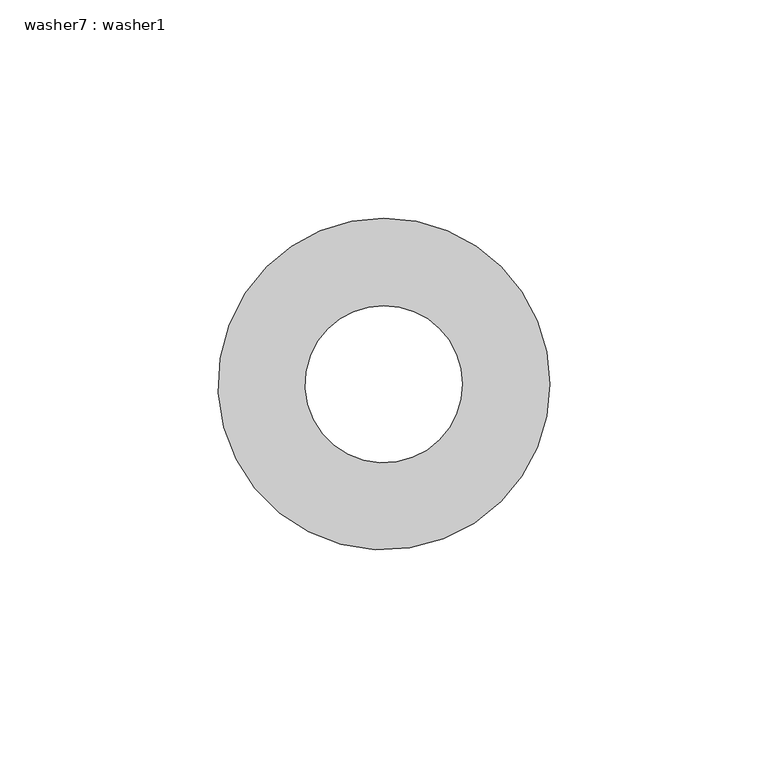
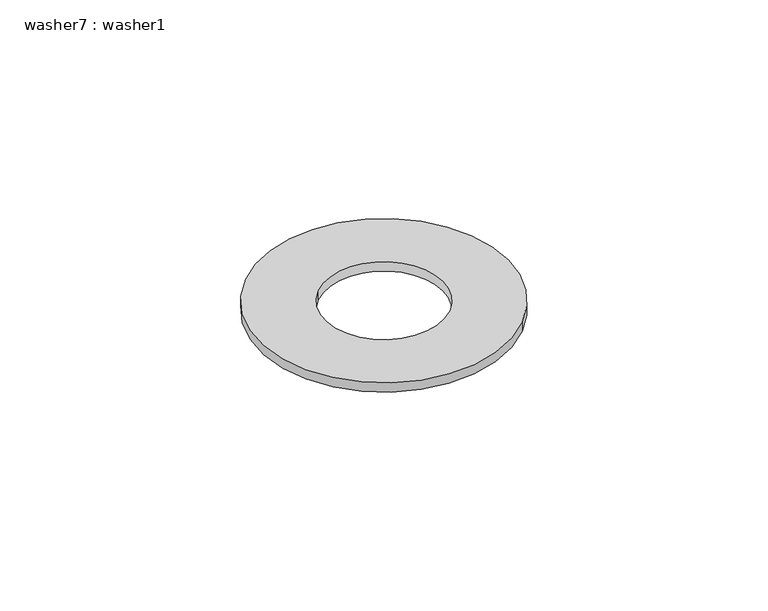
"""IFC4 building model written with IfcOpenShell, lengths in millimetres: fastener geometry, washer7 : washer1."""

import ifcopenshell
import ifcopenshell.guid

model = None  # the IFC model being written
_history = None  # IfcOwnerHistory: only IFC2X3 demands one
_inside = {}  # id of a spatial element -> (the spatial element, [elements in it])
_under = {}  # id of a project, library or spatial element -> (it, [spatial elements below it])
_declared = {}  # id of a project -> (the project, [libraries it declares])
_typed = {}  # id of a type object -> (the type object, [elements of that type])
_made_of = {}  # id of a material, layer set ... -> (it, [elements and type objects made of it])


def new_model(schema):
    """Start an empty IFC model of exactly this schema.

    Asked for "IFC4X3", IfcOpenShell would pick the latest addendum, in which some entities
    have other attributes; the version numbers below select the first issue.
    IFC2X3 requires an IfcOwnerHistory on every rooted entity: one is made here for all.
    """
    global model, _history
    if schema == "IFC4X3":
        model = ifcopenshell.file(schema_version=(4, 3, 0, 0))
    else:
        model = ifcopenshell.file(schema=schema)
    _inside.clear()
    _under.clear()
    _declared.clear()
    _typed.clear()
    _made_of.clear()
    _history = None
    if model.schema == "IFC2X3":
        org = make("IfcOrganization", Name="unknown")
        user = make(
            "IfcPersonAndOrganization",
            ThePerson=make("IfcPerson", FamilyName="unknown"),
            TheOrganization=org,
        )
        app = make(
            "IfcApplication",
            ApplicationDeveloper=org,
            Version="unknown",
            ApplicationFullName="unknown",
            ApplicationIdentifier="unknown",
        )
        _history = make(
            "IfcOwnerHistory",
            OwningUser=user,
            OwningApplication=app,
            ChangeAction="ADDED",
            CreationDate=0,
        )
    return model


def make(cls, **values):
    """One entity of the class cls with the attributes given. An attribute that is None is left unset."""
    return model.create_entity(
        cls, **{name: value for name, value in values.items() if value is not None}
    )


def rooted(cls, **values):
    """An entity with a GlobalId (a new one), such as an element, a storey or a relation."""
    return make(cls, GlobalId=ifcopenshell.guid.new(), OwnerHistory=_history, **values)


def si_unit(unit_type, name, prefix=None):
    """IfcSIUnit, for example si_unit("LENGTHUNIT", "METRE", prefix="MILLI")."""
    return make("IfcSIUnit", UnitType=unit_type, Prefix=prefix, Name=name)


def assignment(units):
    """IfcUnitAssignment: the units of a project."""
    return None if units is None else make("IfcUnitAssignment", Units=units)


def point(xyz):
    """IfcCartesianPoint."""
    return None if xyz is None else make("IfcCartesianPoint", Coordinates=xyz)


def direction(xyz):
    """IfcDirection."""
    return None if xyz is None else make("IfcDirection", DirectionRatios=xyz)


def frame(location, z_axis=None, x_axis=None):
    """IfcAxis2Placement3D, a coordinate frame: its origin and axes. An axis left out is left unset."""
    return make(
        "IfcAxis2Placement3D",
        Location=point(location),
        Axis=direction(z_axis),
        RefDirection=direction(x_axis),
    )


def frame_2d(location, x_axis=None):
    """IfcAxis2Placement2D, a coordinate frame in the plane: its origin and x axis."""
    return make(
        "IfcAxis2Placement2D", Location=point(location), RefDirection=direction(x_axis)
    )


def origin():
    """The frame at (0, 0, 0) with its axes left unset."""
    return frame((0.0, 0.0, 0.0))


def place(relative_to, where):
    """IfcLocalPlacement: puts the frame where relative to a parent placement (None: the world)."""
    return make(
        "IfcLocalPlacement", PlacementRelTo=relative_to, RelativePlacement=where
    )


def context(
    kind, dimensions, precision=None, world=None, true_north=None, identifier=None
):
    """IfcGeometricRepresentationContext, for example the 3D "Model" context."""
    return make(
        "IfcGeometricRepresentationContext",
        ContextIdentifier=identifier,
        ContextType=kind,
        CoordinateSpaceDimension=dimensions,
        Precision=precision,
        WorldCoordinateSystem=world,
        TrueNorth=true_north,
    )


def project(units=None, contexts=None):
    """IfcProject with its units and contexts."""
    return rooted(
        "IfcProject",
        Name="project",
        RepresentationContexts=contexts,
        UnitsInContext=assignment(units),
    )


def spatial(cls, under=None, at=None, **own):
    """A site, building, storey or space (cls), placed at a placement, below another one or the project."""
    s = rooted(cls, ObjectPlacement=at, **own)
    if under is not None:
        _under.setdefault(under.id(), (under, []))[1].append(s)
    return s


def circle_curve(where, radius):
    """IfcCircle in the frame where."""
    return make("IfcCircle", Position=where, Radius=radius)


def trimmed(basis, trim1, trim2, sense, master):
    """IfcTrimmedCurve: the piece of a basis curve between two trims."""
    return make(
        "IfcTrimmedCurve",
        BasisCurve=basis,
        Trim1=trim1,
        Trim2=trim2,
        SenseAgreement=sense,
        MasterRepresentation=master,
    )


def segment(curve, same_sense, transition):
    """IfcCompositeCurveSegment."""
    return make(
        "IfcCompositeCurveSegment",
        Transition=transition,
        SameSense=same_sense,
        ParentCurve=curve,
    )


def composite_curve(segments, self_intersect=None):
    """IfcCompositeCurve: segments joined end to end."""
    return make("IfcCompositeCurve", Segments=segments, SelfIntersect=self_intersect)


def outline(outer, holes=None, kind="AREA"):
    """IfcArbitraryClosedProfileDef: a profile drawn as a closed curve; with holes, ...WithVoids."""
    if holes is None:
        return make("IfcArbitraryClosedProfileDef", ProfileType=kind, OuterCurve=outer)
    return make(
        "IfcArbitraryProfileDefWithVoids",
        ProfileType=kind,
        OuterCurve=outer,
        InnerCurves=holes,
    )


def extrude(swept, where, along, depth):
    """IfcExtrudedAreaSolid: the profile swept, set in the frame where, extruded along a direction by depth."""
    return make(
        "IfcExtrudedAreaSolid",
        SweptArea=swept,
        Position=where,
        ExtrudedDirection=direction(along),
        Depth=depth,
    )


def shape(context_of_items, identifier, shape_type, items):
    """IfcShapeRepresentation: the items that make up one representation, for example the "Body"."""
    return make(
        "IfcShapeRepresentation",
        ContextOfItems=context_of_items,
        RepresentationIdentifier=identifier,
        RepresentationType=shape_type,
        Items=items,
    )


def source(mapping_origin, context_of_items, identifier, shape_type, items):
    """IfcRepresentationMap: a shape defined once, which mapped items show again and again."""
    return make(
        "IfcRepresentationMap",
        MappingOrigin=mapping_origin,
        MappedRepresentation=shape(context_of_items, identifier, shape_type, items),
    )


def transform(
    local_origin,
    x_axis=None,
    y_axis=None,
    z_axis=None,
    scale=None,
    scale2=None,
    scale3=None,
    uniform=True,
):
    """IfcCartesianTransformationOperator3D, or its non-uniform kind. x_axis, y_axis, z_axis: its Axis1, 2, 3."""
    if uniform:
        return make(
            "IfcCartesianTransformationOperator3D",
            Axis1=direction(x_axis),
            Axis2=direction(y_axis),
            LocalOrigin=point(local_origin),
            Scale=scale,
            Axis3=direction(z_axis),
        )
    return make(
        "IfcCartesianTransformationOperator3DnonUniform",
        Axis1=direction(x_axis),
        Axis2=direction(y_axis),
        LocalOrigin=point(local_origin),
        Scale=scale,
        Axis3=direction(z_axis),
        Scale2=scale2,
        Scale3=scale3,
    )


def mapped(mapping_source, mapping_target):
    """IfcMappedItem: shows the shape of a source again, moved by a transform."""
    return make(
        "IfcMappedItem", MappingSource=mapping_source, MappingTarget=mapping_target
    )


def made_of(thing, what):
    """Note that an element or type object is made of a material, layer set ...; save() writes the relation."""
    if what is not None:
        _made_of.setdefault(what.id(), (what, []))[1].append(thing)
    return thing


def element(
    cls,
    number,
    at=None,
    inside=None,
    cuts=None,
    type_object=None,
    material=None,
    context=None,
    identifier="Body",
    shape_type=None,
    held_by="IfcProductDefinitionShape",
    body=None,
    shapes=None,
    **own,
):
    """One element of the class cls, such as IfcWall. Its Tag is "e" and its number.

    at: its placement. inside: the storey or other place that contains it. cuts: it is an
    opening in that element (IfcRelVoidsElement). A single representation is given by context,
    identifier, shape_type and body (its items); several are given by shapes. held_by: the class
    of the entity that holds the representations. save() writes the other relations.
    """
    e = rooted(cls, Tag="e%d" % number, ObjectPlacement=at, **own)
    if body is not None:
        shapes = [shape(context, identifier, shape_type, body)]
    if shapes is not None:
        e.Representation = make(held_by, Representations=shapes)
    if inside is not None:
        _inside.setdefault(inside.id(), (inside, []))[1].append(e)
    if cuts is not None:
        rooted(
            "IfcRelVoidsElement", RelatingBuildingElement=cuts, RelatedOpeningElement=e
        )
    if type_object is not None:
        _typed.setdefault(type_object.id(), (type_object, []))[1].append(e)
    return made_of(e, material)


def aggregate(whole, parts):
    """IfcRelAggregates: a whole, such as a stair, and the parts it consists of."""
    return rooted("IfcRelAggregates", RelatingObject=whole, RelatedObjects=parts)


def save(model, path):
    """Write the relations noted so far, then the file.

    IfcRelAggregates (storeys below a building ...), IfcRelContainedInSpatialStructure (elements
    in a storey), IfcRelDefinesByType, IfcRelAssociatesMaterial and IfcRelDeclares: one each for
    every whole, place, type object, material and project.
    """
    for whole, parts in _under.values():
        aggregate(whole, parts)
    for where, things in _inside.values():
        rooted(
            "IfcRelContainedInSpatialStructure",
            RelatedElements=things,
            RelatingStructure=where,
        )
    for kind, things in _typed.values():
        rooted("IfcRelDefinesByType", RelatedObjects=things, RelatingType=kind)
    for what, things in _made_of.values():
        rooted("IfcRelAssociatesMaterial", RelatedObjects=things, RelatingMaterial=what)
    for by, libraries in _declared.values():
        rooted("IfcRelDeclares", RelatingContext=by, RelatedDefinitions=libraries)
    model.write(path)


def washer7_washer1_ec282568(model_context):
    return source(origin(), model_context, "Body", "SweptSolid", [
        extrude(outline(composite_curve([segment(trimmed(circle_curve(frame_2d((-31212.5323938, -7850.7265865)), 38.0), [point((-31239.4024515, -7823.8565288))], [point((-31185.6623362, -7877.5966442))], False, "CARTESIAN"), True, "CONTINUOUS"), segment(trimmed(circle_curve(frame_2d((-31212.5323938, -7850.7265865)), 38.0), [point((-31185.6623362, -7877.5966442))], [point((-31239.4024515, -7823.8565288))], False, "CARTESIAN"), True, "CONTINUOUS")], self_intersect=False), holes=[composite_curve([segment(trimmed(circle_curve(frame_2d((-31212.5323938, -7850.7265865)), 18.0), [point((-31225.2603159, -7837.9986645))], [point((-31199.8044718, -7863.4545086))], True, "CARTESIAN"), True, "CONTINUOUS"), segment(trimmed(circle_curve(frame_2d((-31212.5323938, -7850.7265865)), 18.0), [point((-31199.8044718, -7863.4545086))], [point((-31225.2603159, -7837.9986645))], True, "CARTESIAN"), True, "CONTINUOUS")], self_intersect=False)]), frame((0.0, 0.0, 117.0), z_axis=(0.0, 0.0, 1.0), x_axis=(1.0, 0.0, 0.0)), (0.0, 0.0, 1.0), 3.0),
    ])


if __name__ == "__main__":
    model = new_model("IFC4")
    model_context = context("Model", 3, world=origin())
    ifc_project = project(units=[si_unit("LENGTHUNIT", "METRE", prefix="MILLI")], contexts=[model_context])
    site = spatial("IfcSite", under=ifc_project)
    building = spatial("IfcBuilding", under=site)
    placement = place(None, origin())
    washer7_washer1_shape = washer7_washer1_ec282568(model_context)
    element("IfcFastener", 1, ObjectType="washer7 : washer1", at=placement, inside=building, context=model_context, shape_type="MappedRepresentation", body=[
        mapped(washer7_washer1_shape, transform((0.0, 0.0, 0.0), x_axis=(1.0, 0.0, 0.0), y_axis=(0.0, 1.0, 0.0), z_axis=(0.0, 0.0, 1.0))),
    ])
    save(model, "model.ifc")

# Revit data of these elements
# Element 1 (IfcFastener, "washer7 : washer1")
#   Materials on its faces: "A05ZZ166-00007_Roof_Sandiwch Panel_Mineral Wool_non FP"
# Materials
#   "A05ZZ166-00007_Roof_Sandiwch Panel_Mineral Wool_non FP": class "*O 수장공사 - 패널", colour RGB 242 242 242, transparency 0, Keynote = "OJ4", Description = "샌드위치패널", W00) Work Master Code = "A05ZZ166-00007", W01) Work Master_Lv1 = "Cladding Work", W02) Work Master_Lv2 = "Sandwich Panel", W03) Work Master_Spec.1 = "Corrugated Galvanized Steel Sheet Sandwich Panel, Fire Protective Rating: N/A", W04) Work Master_Spec.2 = "Mineral Wool", W05) Work Master_Spec.3 = "w/ Accessories, Flashing", W06) Work Master_Spec.4 = "100mm≤THK<150mm", Cost = 0
